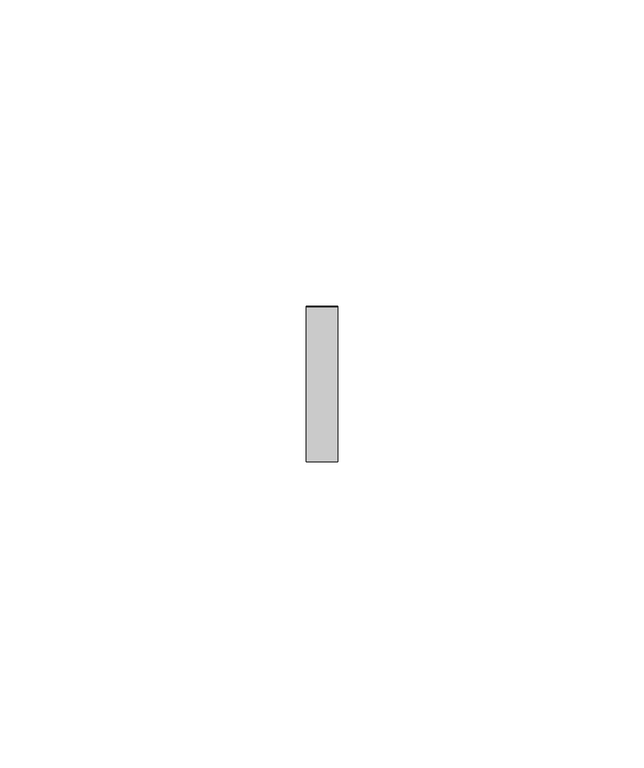
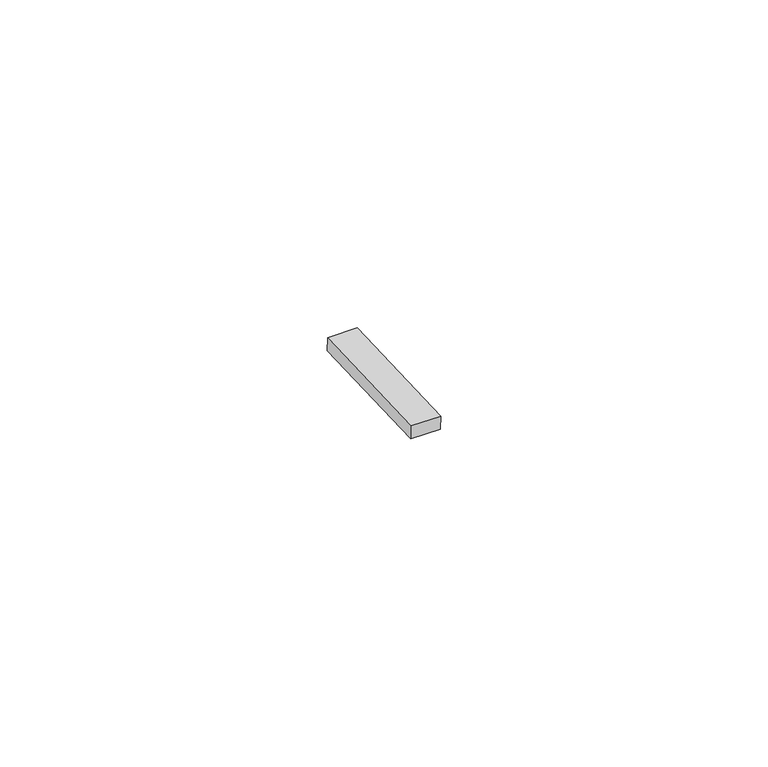
"""IFC4 building model written with IfcOpenShell, lengths in millimetres: proxy geometry, Inner panel:Inner panel:1:Inner panel:1 : Inner panel:Inner panel:300324:2:Inner panel:1:Inner panel:1 : Inner panel:Inner panel:300324:2 : Inner panel:Inner panel:1:Inner panel:1 : Inner panel:Inner panel:300324:300043:64 : Inner panel:Inner panel:1:Inner panel:1 : Inner panel:Inner panel:300324:2:Inner panel:1:Inner panel:1 : Inner panel:Inner panel:300324:2 : Inner panel:Inner panel:1:Inner panel:1 : Inner panel:Inner panel:300324:300043:308120."""

import ifcopenshell
import ifcopenshell.guid

model = None  # the IFC model being written
_history = None  # IfcOwnerHistory: only IFC2X3 demands one
_inside = {}  # id of a spatial element -> (the spatial element, [elements in it])
_under = {}  # id of a project, library or spatial element -> (it, [spatial elements below it])
_declared = {}  # id of a project -> (the project, [libraries it declares])
_typed = {}  # id of a type object -> (the type object, [elements of that type])
_made_of = {}  # id of a material, layer set ... -> (it, [elements and type objects made of it])


def new_model(schema):
    """Start an empty IFC model of exactly this schema.

    Asked for "IFC4X3", IfcOpenShell would pick the latest addendum, in which some entities
    have other attributes; the version numbers below select the first issue.
    IFC2X3 requires an IfcOwnerHistory on every rooted entity: one is made here for all.
    """
    global model, _history
    if schema == "IFC4X3":
        model = ifcopenshell.file(schema_version=(4, 3, 0, 0))
    else:
        model = ifcopenshell.file(schema=schema)
    _inside.clear()
    _under.clear()
    _declared.clear()
    _typed.clear()
    _made_of.clear()
    _history = None
    if model.schema == "IFC2X3":
        org = make("IfcOrganization", Name="unknown")
        user = make(
            "IfcPersonAndOrganization",
            ThePerson=make("IfcPerson", FamilyName="unknown"),
            TheOrganization=org,
        )
        app = make(
            "IfcApplication",
            ApplicationDeveloper=org,
            Version="unknown",
            ApplicationFullName="unknown",
            ApplicationIdentifier="unknown",
        )
        _history = make(
            "IfcOwnerHistory",
            OwningUser=user,
            OwningApplication=app,
            ChangeAction="ADDED",
            CreationDate=0,
        )
    return model


def make(cls, **values):
    """One entity of the class cls with the attributes given. An attribute that is None is left unset."""
    return model.create_entity(
        cls, **{name: value for name, value in values.items() if value is not None}
    )


def rooted(cls, **values):
    """An entity with a GlobalId (a new one), such as an element, a storey or a relation."""
    return make(cls, GlobalId=ifcopenshell.guid.new(), OwnerHistory=_history, **values)


def si_unit(unit_type, name, prefix=None):
    """IfcSIUnit, for example si_unit("LENGTHUNIT", "METRE", prefix="MILLI")."""
    return make("IfcSIUnit", UnitType=unit_type, Prefix=prefix, Name=name)


def assignment(units):
    """IfcUnitAssignment: the units of a project."""
    return None if units is None else make("IfcUnitAssignment", Units=units)


def point(xyz):
    """IfcCartesianPoint."""
    return None if xyz is None else make("IfcCartesianPoint", Coordinates=xyz)


def direction(xyz):
    """IfcDirection."""
    return None if xyz is None else make("IfcDirection", DirectionRatios=xyz)


def frame(location, z_axis=None, x_axis=None):
    """IfcAxis2Placement3D, a coordinate frame: its origin and axes. An axis left out is left unset."""
    return make(
        "IfcAxis2Placement3D",
        Location=point(location),
        Axis=direction(z_axis),
        RefDirection=direction(x_axis),
    )


def origin():
    """The frame at (0, 0, 0) with its axes left unset."""
    return frame((0.0, 0.0, 0.0))


def place(relative_to, where):
    """IfcLocalPlacement: puts the frame where relative to a parent placement (None: the world)."""
    return make(
        "IfcLocalPlacement", PlacementRelTo=relative_to, RelativePlacement=where
    )


def context(
    kind, dimensions, precision=None, world=None, true_north=None, identifier=None
):
    """IfcGeometricRepresentationContext, for example the 3D "Model" context."""
    return make(
        "IfcGeometricRepresentationContext",
        ContextIdentifier=identifier,
        ContextType=kind,
        CoordinateSpaceDimension=dimensions,
        Precision=precision,
        WorldCoordinateSystem=world,
        TrueNorth=true_north,
    )


def project(units=None, contexts=None):
    """IfcProject with its units and contexts."""
    return rooted(
        "IfcProject",
        Name="project",
        RepresentationContexts=contexts,
        UnitsInContext=assignment(units),
    )


def spatial(cls, under=None, at=None, **own):
    """A site, building, storey or space (cls), placed at a placement, below another one or the project."""
    s = rooted(cls, ObjectPlacement=at, **own)
    if under is not None:
        _under.setdefault(under.id(), (under, []))[1].append(s)
    return s


def polyline(points):
    """IfcPolyline through the points."""
    return make("IfcPolyline", Points=[point(p) for p in points])


def outline(outer, holes=None, kind="AREA"):
    """IfcArbitraryClosedProfileDef: a profile drawn as a closed curve; with holes, ...WithVoids."""
    if holes is None:
        return make("IfcArbitraryClosedProfileDef", ProfileType=kind, OuterCurve=outer)
    return make(
        "IfcArbitraryProfileDefWithVoids",
        ProfileType=kind,
        OuterCurve=outer,
        InnerCurves=holes,
    )


def extrude(swept, where, along, depth):
    """IfcExtrudedAreaSolid: the profile swept, set in the frame where, extruded along a direction by depth."""
    return make(
        "IfcExtrudedAreaSolid",
        SweptArea=swept,
        Position=where,
        ExtrudedDirection=direction(along),
        Depth=depth,
    )


def shape(context_of_items, identifier, shape_type, items):
    """IfcShapeRepresentation: the items that make up one representation, for example the "Body"."""
    return make(
        "IfcShapeRepresentation",
        ContextOfItems=context_of_items,
        RepresentationIdentifier=identifier,
        RepresentationType=shape_type,
        Items=items,
    )


def source(mapping_origin, context_of_items, identifier, shape_type, items):
    """IfcRepresentationMap: a shape defined once, which mapped items show again and again."""
    return make(
        "IfcRepresentationMap",
        MappingOrigin=mapping_origin,
        MappedRepresentation=shape(context_of_items, identifier, shape_type, items),
    )


def transform(
    local_origin,
    x_axis=None,
    y_axis=None,
    z_axis=None,
    scale=None,
    scale2=None,
    scale3=None,
    uniform=True,
):
    """IfcCartesianTransformationOperator3D, or its non-uniform kind. x_axis, y_axis, z_axis: its Axis1, 2, 3."""
    if uniform:
        return make(
            "IfcCartesianTransformationOperator3D",
            Axis1=direction(x_axis),
            Axis2=direction(y_axis),
            LocalOrigin=point(local_origin),
            Scale=scale,
            Axis3=direction(z_axis),
        )
    return make(
        "IfcCartesianTransformationOperator3DnonUniform",
        Axis1=direction(x_axis),
        Axis2=direction(y_axis),
        LocalOrigin=point(local_origin),
        Scale=scale,
        Axis3=direction(z_axis),
        Scale2=scale2,
        Scale3=scale3,
    )


def mapped(mapping_source, mapping_target):
    """IfcMappedItem: shows the shape of a source again, moved by a transform."""
    return make(
        "IfcMappedItem", MappingSource=mapping_source, MappingTarget=mapping_target
    )


def made_of(thing, what):
    """Note that an element or type object is made of a material, layer set ...; save() writes the relation."""
    if what is not None:
        _made_of.setdefault(what.id(), (what, []))[1].append(thing)
    return thing


def element(
    cls,
    number,
    at=None,
    inside=None,
    cuts=None,
    type_object=None,
    material=None,
    context=None,
    identifier="Body",
    shape_type=None,
    held_by="IfcProductDefinitionShape",
    body=None,
    shapes=None,
    **own,
):
    """One element of the class cls, such as IfcWall. Its Tag is "e" and its number.

    at: its placement. inside: the storey or other place that contains it. cuts: it is an
    opening in that element (IfcRelVoidsElement). A single representation is given by context,
    identifier, shape_type and body (its items); several are given by shapes. held_by: the class
    of the entity that holds the representations. save() writes the other relations.
    """
    e = rooted(cls, Tag="e%d" % number, ObjectPlacement=at, **own)
    if body is not None:
        shapes = [shape(context, identifier, shape_type, body)]
    if shapes is not None:
        e.Representation = make(held_by, Representations=shapes)
    if inside is not None:
        _inside.setdefault(inside.id(), (inside, []))[1].append(e)
    if cuts is not None:
        rooted(
            "IfcRelVoidsElement", RelatingBuildingElement=cuts, RelatedOpeningElement=e
        )
    if type_object is not None:
        _typed.setdefault(type_object.id(), (type_object, []))[1].append(e)
    return made_of(e, material)


def aggregate(whole, parts):
    """IfcRelAggregates: a whole, such as a stair, and the parts it consists of."""
    return rooted("IfcRelAggregates", RelatingObject=whole, RelatedObjects=parts)


def save(model, path):
    """Write the relations noted so far, then the file.

    IfcRelAggregates (storeys below a building ...), IfcRelContainedInSpatialStructure (elements
    in a storey), IfcRelDefinesByType, IfcRelAssociatesMaterial and IfcRelDeclares: one each for
    every whole, place, type object, material and project.
    """
    for whole, parts in _under.values():
        aggregate(whole, parts)
    for where, things in _inside.values():
        rooted(
            "IfcRelContainedInSpatialStructure",
            RelatedElements=things,
            RelatingStructure=where,
        )
    for kind, things in _typed.values():
        rooted("IfcRelDefinesByType", RelatedObjects=things, RelatingType=kind)
    for what, things in _made_of.values():
        rooted("IfcRelAssociatesMaterial", RelatedObjects=things, RelatingMaterial=what)
    for by, libraries in _declared.values():
        rooted("IfcRelDeclares", RelatingContext=by, RelatedDefinitions=libraries)
    model.write(path)


def generic_models_cbd9dd92(model_context):
    return source(origin(), model_context, "Body", "SweptSolid", [
        extrude(outline(polyline([(0.0, -25.3999999), (0.0, 0.0), (5.2138089, 0.0), (5.2138089, -25.3999999), (0.0, -25.3999999)])), frame((593123.795117, -566905.6162814, 8857.0720004), z_axis=(0.0, -0.041630544712223896, 0.9991330730923502), x_axis=(-1.0, 0.0, 0.0)), (0.0, 0.0, 1.0), 2.4763745),
    ])


if __name__ == "__main__":
    model = new_model("IFC4")
    model_context = context("Model", 3, world=origin())
    ifc_project = project(units=[si_unit("LENGTHUNIT", "METRE", prefix="MILLI")], contexts=[model_context])
    site = spatial("IfcSite", under=ifc_project)
    building = spatial("IfcBuilding", under=site)
    placement = place(None, origin())
    generic_models_shape = generic_models_cbd9dd92(model_context)
    element("IfcBuildingElementProxy", 1, Name="Inner panel:Inner panel:1:Inner panel:1 : Inner panel:Inner panel:300324:2:Inner panel:1:Inner panel:1 : Inner panel:Inner panel:300324:2 : Inner panel:Inner panel:1:Inner panel:1 : Inner panel:Inner panel:300324:300043:64 : Inner panel:Inner panel:1:Inner panel:1 : Inner panel:Inner panel:300324:2:Inner panel:1:Inner panel:1 : Inner panel:Inner panel:300324:2 : Inner panel:Inner panel:1:Inner panel:1 : Inner panel:Inner panel:300324:300043:308120", ObjectType="Inner panel:Inner panel:1:Inner panel:1 : Inner panel:Inner panel:300324:2:Inner panel:1:Inner panel:1 : Inner panel:Inner panel:300324:2 : Inner panel:Inner panel:1:Inner panel:1 : Inner panel:Inner panel:300324:300043:64 : Inner panel:Inner panel:1:Inner panel:1 : Inner panel:Inner panel:300324:2:Inner panel:1:Inner panel:1 : Inner panel:Inner panel:300324:2 : Inner panel:Inner panel:1:Inner panel:1 : Inner panel:Inner panel:300324:300043:308120", at=placement, inside=building, context=model_context, shape_type="MappedRepresentation", body=[
        mapped(generic_models_shape, transform((0.0, 0.0, 0.0), x_axis=(1.0, 0.0, 0.0), y_axis=(0.0, 1.0, 0.0), z_axis=(0.0, 0.0, 1.0))),
    ])
    save(model, "model.ifc")

# Revit data of these elements
# Type "Inner panel:Inner panel:1:Inner panel:1 : Inner panel:Inner panel:300324:2:Inner panel:1:Inner panel:1 : Inner panel:Inner panel:300324:2 : Inner panel:Inner panel:1:Inner panel:1 : Inner panel:Inner panel:300324:300043:64 : Inner panel:Inner panel:1:Inner panel:1 : Inner panel:Inner panel:300324:2:Inner panel:1:Inner panel:1 : Inner panel:Inner panel:300324:2 : Inner panel:Inner panel:1:Inner panel:1 : Inner panel:Inner panel:300324:300043:308120"
#   NameOverride = "Inner panel:Inner panel:1:Inner panel:1 : Inner panel:Inner panel:300324:2:Inner panel:1:Inner panel:1 : Inner panel:Inner panel:300324:2 : Inner panel:Inner panel:1:Inner panel:1 : Inner panel:Inner panel:300324:300043:308120"
#   ObjectTypeOverride = "Inner panel:1:Inner panel:1 : Inner panel:Inner panel:300324:2 : Inner panel:Inner panel:1:Inner panel:1 : Inner panel:Inner panel:300324:300043"
#   Reference = "Inner panel"
#   Tag = "308120"
# Element 1 (IfcBuildingElementProxy, "Inner panel:Inner panel:1:Inner panel:1 : Inner panel:Inner panel:300324:2:Inner panel:1:Inner panel:1 : Inner panel:Inner panel:300324:2 : Inner panel:Inner panel:1:Inner panel:1 : Inner panel:Inner panel:300324:300043:64 : Inner panel:Inner panel:1:Inner panel:1 : Inner panel:Inner panel:300324:2:Inner panel:1:Inner panel:1 : Inner panel:Inner panel:300324:2 : Inner panel:Inner panel:1:Inner panel:1 : Inner panel:Inner panel:300324:300043:308120")
#   Materials on its faces: "AT CLIP - 1\" WIDE NON ABSORBENT, WEATHER-RESISTANT NEOPRENE/EPDM/SBR FOAM"
# Materials
#   "AT CLIP - 1\" WIDE NON ABSORBENT, WEATHER-RESISTANT NEOPRENE/EPDM/SBR FOAM": class "Generic", colour RGB 85 85 85, transparency 0, Cost = 0
